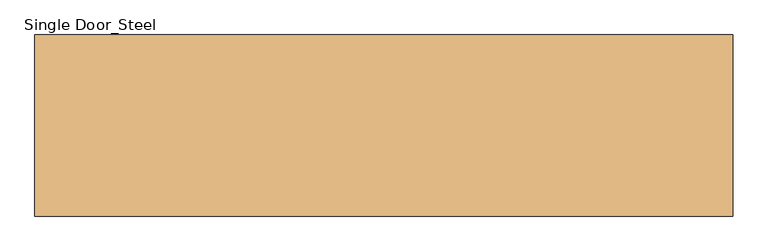
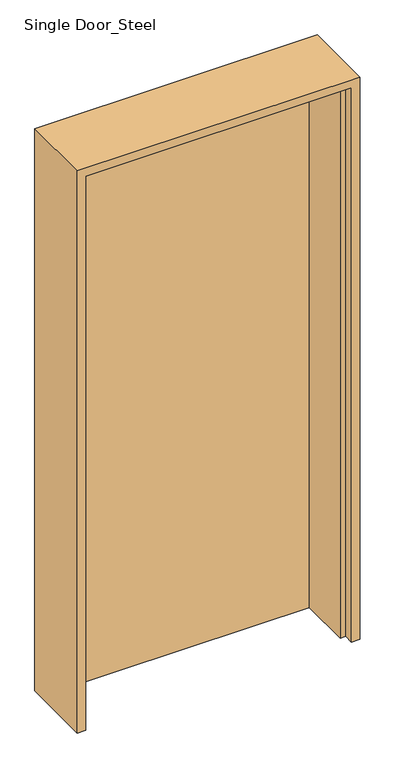
"""IFC4 building model written with IfcOpenShell, lengths in millimetres: door geometry, Single Door_Steel : H_DR_AR_B12_Single Door_Steel_W1000xH2100."""

import ifcopenshell
import ifcopenshell.guid

model = None  # the IFC model being written
_history = None  # IfcOwnerHistory: only IFC2X3 demands one
_inside = {}  # id of a spatial element -> (the spatial element, [elements in it])
_under = {}  # id of a project, library or spatial element -> (it, [spatial elements below it])
_declared = {}  # id of a project -> (the project, [libraries it declares])
_typed = {}  # id of a type object -> (the type object, [elements of that type])
_made_of = {}  # id of a material, layer set ... -> (it, [elements and type objects made of it])


def new_model(schema):
    """Start an empty IFC model of exactly this schema.

    Asked for "IFC4X3", IfcOpenShell would pick the latest addendum, in which some entities
    have other attributes; the version numbers below select the first issue.
    IFC2X3 requires an IfcOwnerHistory on every rooted entity: one is made here for all.
    """
    global model, _history
    if schema == "IFC4X3":
        model = ifcopenshell.file(schema_version=(4, 3, 0, 0))
    else:
        model = ifcopenshell.file(schema=schema)
    _inside.clear()
    _under.clear()
    _declared.clear()
    _typed.clear()
    _made_of.clear()
    _history = None
    if model.schema == "IFC2X3":
        org = make("IfcOrganization", Name="unknown")
        user = make(
            "IfcPersonAndOrganization",
            ThePerson=make("IfcPerson", FamilyName="unknown"),
            TheOrganization=org,
        )
        app = make(
            "IfcApplication",
            ApplicationDeveloper=org,
            Version="unknown",
            ApplicationFullName="unknown",
            ApplicationIdentifier="unknown",
        )
        _history = make(
            "IfcOwnerHistory",
            OwningUser=user,
            OwningApplication=app,
            ChangeAction="ADDED",
            CreationDate=0,
        )
    return model


def make(cls, **values):
    """One entity of the class cls with the attributes given. An attribute that is None is left unset."""
    return model.create_entity(
        cls, **{name: value for name, value in values.items() if value is not None}
    )


def rooted(cls, **values):
    """An entity with a GlobalId (a new one), such as an element, a storey or a relation."""
    return make(cls, GlobalId=ifcopenshell.guid.new(), OwnerHistory=_history, **values)


def si_unit(unit_type, name, prefix=None):
    """IfcSIUnit, for example si_unit("LENGTHUNIT", "METRE", prefix="MILLI")."""
    return make("IfcSIUnit", UnitType=unit_type, Prefix=prefix, Name=name)


def assignment(units):
    """IfcUnitAssignment: the units of a project."""
    return None if units is None else make("IfcUnitAssignment", Units=units)


def point(xyz):
    """IfcCartesianPoint."""
    return None if xyz is None else make("IfcCartesianPoint", Coordinates=xyz)


def direction(xyz):
    """IfcDirection."""
    return None if xyz is None else make("IfcDirection", DirectionRatios=xyz)


def frame(location, z_axis=None, x_axis=None):
    """IfcAxis2Placement3D, a coordinate frame: its origin and axes. An axis left out is left unset."""
    return make(
        "IfcAxis2Placement3D",
        Location=point(location),
        Axis=direction(z_axis),
        RefDirection=direction(x_axis),
    )


def origin():
    """The frame at (0, 0, 0) with its axes left unset."""
    return frame((0.0, 0.0, 0.0))


def origin_with_axes():
    """The frame at (0, 0, 0) with the z axis (0, 0, 1) and the x axis (1, 0, 0) written out."""
    return frame((0.0, 0.0, 0.0), z_axis=(0.0, 0.0, 1.0), x_axis=(1.0, 0.0, 0.0))


def place(relative_to, where):
    """IfcLocalPlacement: puts the frame where relative to a parent placement (None: the world)."""
    return make(
        "IfcLocalPlacement", PlacementRelTo=relative_to, RelativePlacement=where
    )


def context(
    kind, dimensions, precision=None, world=None, true_north=None, identifier=None
):
    """IfcGeometricRepresentationContext, for example the 3D "Model" context."""
    return make(
        "IfcGeometricRepresentationContext",
        ContextIdentifier=identifier,
        ContextType=kind,
        CoordinateSpaceDimension=dimensions,
        Precision=precision,
        WorldCoordinateSystem=world,
        TrueNorth=true_north,
    )


def project(units=None, contexts=None):
    """IfcProject with its units and contexts."""
    return rooted(
        "IfcProject",
        Name="project",
        RepresentationContexts=contexts,
        UnitsInContext=assignment(units),
    )


def spatial(cls, under=None, at=None, **own):
    """A site, building, storey or space (cls), placed at a placement, below another one or the project."""
    s = rooted(cls, ObjectPlacement=at, **own)
    if under is not None:
        _under.setdefault(under.id(), (under, []))[1].append(s)
    return s


def polyline(points):
    """IfcPolyline through the points."""
    return make("IfcPolyline", Points=[point(p) for p in points])


def outline(outer, holes=None, kind="AREA"):
    """IfcArbitraryClosedProfileDef: a profile drawn as a closed curve; with holes, ...WithVoids."""
    if holes is None:
        return make("IfcArbitraryClosedProfileDef", ProfileType=kind, OuterCurve=outer)
    return make(
        "IfcArbitraryProfileDefWithVoids",
        ProfileType=kind,
        OuterCurve=outer,
        InnerCurves=holes,
    )


def extrude(swept, where, along, depth):
    """IfcExtrudedAreaSolid: the profile swept, set in the frame where, extruded along a direction by depth."""
    return make(
        "IfcExtrudedAreaSolid",
        SweptArea=swept,
        Position=where,
        ExtrudedDirection=direction(along),
        Depth=depth,
    )


def faces_of(points, faces, orient=None, outer=None):
    """IfcFace entities. A face is a list of loops; a loop is a list of indices into points, from 0.

    orient and outer hold one flag for each loop. By default every Orientation is true, the
    first loop of a face is its IfcFaceOuterBound and the others are IfcFaceBound.
    """
    made = []
    for i, loops in enumerate(faces):
        bounds = []
        for j, loop in enumerate(loops):
            is_outer = j == 0 if outer is None else outer[i][j]
            bounds.append(
                make(
                    "IfcFaceOuterBound" if is_outer else "IfcFaceBound",
                    Bound=make("IfcPolyLoop", Polygon=[points[k] for k in loop]),
                    Orientation=True if orient is None else orient[i][j],
                )
            )
        made.append(make("IfcFace", Bounds=bounds))
    return made


def faceted_brep(points, faces, orient=None, outer=None, voids=None):
    """IfcFacetedBrep: a solid bounded by flat faces; with voids (closed shells), ...WithVoids."""
    shared = [point(p) for p in points]
    hull = make("IfcClosedShell", CfsFaces=faces_of(shared, faces, orient, outer))
    if voids is None:
        return make("IfcFacetedBrep", Outer=hull)
    return make(
        "IfcFacetedBrepWithVoids",
        Outer=hull,
        Voids=[
            make(cls, CfsFaces=faces_of(shared, fs, o, b)) for cls, fs, o, b in voids
        ],
    )


def shape(context_of_items, identifier, shape_type, items):
    """IfcShapeRepresentation: the items that make up one representation, for example the "Body"."""
    return make(
        "IfcShapeRepresentation",
        ContextOfItems=context_of_items,
        RepresentationIdentifier=identifier,
        RepresentationType=shape_type,
        Items=items,
    )


def source(mapping_origin, context_of_items, identifier, shape_type, items):
    """IfcRepresentationMap: a shape defined once, which mapped items show again and again."""
    return make(
        "IfcRepresentationMap",
        MappingOrigin=mapping_origin,
        MappedRepresentation=shape(context_of_items, identifier, shape_type, items),
    )


def transform(
    local_origin,
    x_axis=None,
    y_axis=None,
    z_axis=None,
    scale=None,
    scale2=None,
    scale3=None,
    uniform=True,
):
    """IfcCartesianTransformationOperator3D, or its non-uniform kind. x_axis, y_axis, z_axis: its Axis1, 2, 3."""
    if uniform:
        return make(
            "IfcCartesianTransformationOperator3D",
            Axis1=direction(x_axis),
            Axis2=direction(y_axis),
            LocalOrigin=point(local_origin),
            Scale=scale,
            Axis3=direction(z_axis),
        )
    return make(
        "IfcCartesianTransformationOperator3DnonUniform",
        Axis1=direction(x_axis),
        Axis2=direction(y_axis),
        LocalOrigin=point(local_origin),
        Scale=scale,
        Axis3=direction(z_axis),
        Scale2=scale2,
        Scale3=scale3,
    )


def mapped(mapping_source, mapping_target):
    """IfcMappedItem: shows the shape of a source again, moved by a transform."""
    return make(
        "IfcMappedItem", MappingSource=mapping_source, MappingTarget=mapping_target
    )


def made_of(thing, what):
    """Note that an element or type object is made of a material, layer set ...; save() writes the relation."""
    if what is not None:
        _made_of.setdefault(what.id(), (what, []))[1].append(thing)
    return thing


def element(
    cls,
    number,
    at=None,
    inside=None,
    cuts=None,
    type_object=None,
    material=None,
    context=None,
    identifier="Body",
    shape_type=None,
    held_by="IfcProductDefinitionShape",
    body=None,
    shapes=None,
    **own,
):
    """One element of the class cls, such as IfcWall. Its Tag is "e" and its number.

    at: its placement. inside: the storey or other place that contains it. cuts: it is an
    opening in that element (IfcRelVoidsElement). A single representation is given by context,
    identifier, shape_type and body (its items); several are given by shapes. held_by: the class
    of the entity that holds the representations. save() writes the other relations.
    """
    e = rooted(cls, Tag="e%d" % number, ObjectPlacement=at, **own)
    if body is not None:
        shapes = [shape(context, identifier, shape_type, body)]
    if shapes is not None:
        e.Representation = make(held_by, Representations=shapes)
    if inside is not None:
        _inside.setdefault(inside.id(), (inside, []))[1].append(e)
    if cuts is not None:
        rooted(
            "IfcRelVoidsElement", RelatingBuildingElement=cuts, RelatedOpeningElement=e
        )
    if type_object is not None:
        _typed.setdefault(type_object.id(), (type_object, []))[1].append(e)
    return made_of(e, material)


def aggregate(whole, parts):
    """IfcRelAggregates: a whole, such as a stair, and the parts it consists of."""
    return rooted("IfcRelAggregates", RelatingObject=whole, RelatedObjects=parts)


def save(model, path):
    """Write the relations noted so far, then the file.

    IfcRelAggregates (storeys below a building ...), IfcRelContainedInSpatialStructure (elements
    in a storey), IfcRelDefinesByType, IfcRelAssociatesMaterial and IfcRelDeclares: one each for
    every whole, place, type object, material and project.
    """
    for whole, parts in _under.values():
        aggregate(whole, parts)
    for where, things in _inside.values():
        rooted(
            "IfcRelContainedInSpatialStructure",
            RelatedElements=things,
            RelatingStructure=where,
        )
    for kind, things in _typed.values():
        rooted("IfcRelDefinesByType", RelatedObjects=things, RelatingType=kind)
    for what, things in _made_of.values():
        rooted("IfcRelAssociatesMaterial", RelatedObjects=things, RelatingMaterial=what)
    for by, libraries in _declared.values():
        rooted("IfcRelDeclares", RelatingContext=by, RelatedDefinitions=libraries)
    model.write(path)


def single_door_steel_4a6c7de9(model_context):
    return source(origin(), model_context, "Body", "SolidModel", [
        extrude(outline(polyline([(470.0, 130.0), (470.0, 95.0), (-470.0, 95.0), (-470.0, 130.0), (470.0, 130.0)])), origin_with_axes(), (0.0, 0.0, 1.0), 2070.0),
        faceted_brep([(470.0, 130.0, 0.0), (500.0, 130.0, 0.0), (500.0, -130.0, 0.0), (470.0, -130.0, 0.0), (470.0, -95.0, 0.0), (450.0, -95.0, 0.0), (450.0, 95.0, 0.0), (470.0, 95.0, 0.0), (470.0, 130.0, 2070.0), (-470.0, 130.0, 2070.0), (-470.0, 130.0, 0.0), (-500.0, 130.0, 0.0), (-500.0, 130.0, 2100.0), (500.0, 130.0, 2100.0), (500.0, -130.0, 2100.0), (-500.0, -130.0, 2100.0), (-500.0, -130.0, 0.0), (-470.0, -130.0, 0.0), (-470.0, -130.0, 2070.0), (470.0, -130.0, 2070.0), (470.0, -95.0, 2070.0), (-470.0, -95.0, 2070.0), (-470.0, -95.0, 0.0), (-450.0, -95.0, 0.0), (-450.0, -95.0, 2050.0), (450.0, -95.0, 2050.0), (450.0, 95.0, 2050.0), (-450.0, 95.0, 2050.0), (-450.0, 95.0, 0.0), (-470.0, 95.0, 0.0), (-470.0, 95.0, 2070.0), (470.0, 95.0, 2070.0)], [[[0, 1, 2, 3, 4, 5, 6, 7]], [[1, 0, 8, 9, 10, 11, 12, 13]], [[2, 1, 13, 14]], [[3, 2, 14, 15, 16, 17, 18, 19]], [[4, 3, 19, 20]], [[5, 4, 20, 21, 22, 23, 24, 25]], [[6, 5, 25, 26]], [[7, 6, 26, 27, 28, 29, 30, 31]], [[0, 7, 31, 8]], [[9, 30, 29, 10]], [[10, 29, 28, 23, 22, 17, 16, 11]], [[15, 12, 11, 16]], [[21, 18, 17, 22]], [[27, 24, 23, 28]], [[14, 13, 12, 15]], [[20, 19, 18, 21]], [[26, 25, 24, 27]], [[8, 31, 30, 9]]]),
    ])


if __name__ == "__main__":
    model = new_model("IFC4")
    model_context = context("Model", 3, world=origin())
    ifc_project = project(units=[si_unit("LENGTHUNIT", "METRE", prefix="MILLI")], contexts=[model_context])
    site = spatial("IfcSite", under=ifc_project)
    building = spatial("IfcBuilding", under=site)
    placement = place(None, origin())
    single_door_steel_shape = single_door_steel_4a6c7de9(model_context)
    element("IfcDoor", 1, ObjectType="Single Door_Steel : H_DR_AR_B12_Single Door_Steel_W1000xH2100", at=placement, inside=building, context=model_context, shape_type="MappedRepresentation", body=[
        mapped(single_door_steel_shape, transform((0.0, 0.0, 0.0), x_axis=(1.0, 0.0, 0.0), y_axis=(0.0, 1.0, 0.0), z_axis=(0.0, 0.0, 1.0))),
    ])
    save(model, "model.ifc")

# Revit data of these elements
# Type "Single Door_Steel : H_DR_AR_B12_Single Door_Steel_W1000xH2100"
#   Type Mark = "SD"
#   Analytic Construction = "<None>"
#   프레임 투영 외부. = 25 mm
#   프레임 투영 내부. = 25 mm
#   프레임 폭 = 75 mm
#   Height = 2100 mm
#   Width = 1000 mm
#   Define Thermal Properties by = 1
#   문 패널 = none
#   문 프레임 = none
#   Function = (empty or 0)
#   Wall Closure = (empty or 0)
